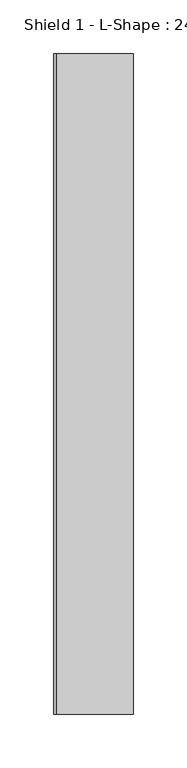
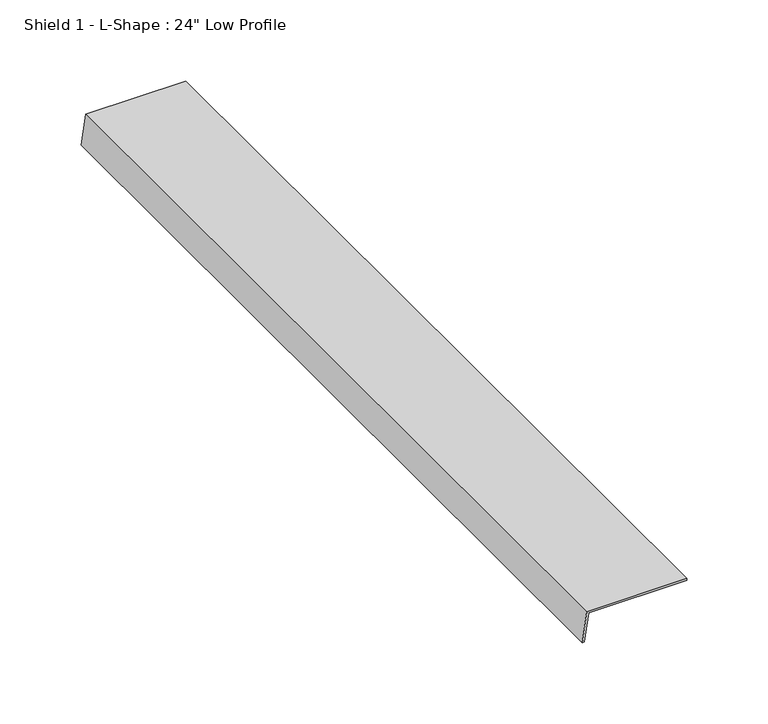
"""IFC4 building model written with IfcOpenShell, lengths in millimetres: proxy geometry."""

from ifc_helpers import new_model, si_unit, frame, origin, place, context, project, spatial, polyline, outline, extrude, source, transform, mapped, element, save


def proxy_87e85a14(model_context):
    return source(origin(), model_context, "Body", "SweptSolid", [
        extrude(outline(polyline([(22.225, -11.0820157), (0.0, -14.2570157), (0.0, -12.6695157), (20.6375, -9.4945157), (20.6375, 60.3554843), (22.225, 60.3554843), (22.225, -11.0820157)])), frame((0.0, -308.76875, 0.0), z_axis=(0.0, 1.0, 0.0), x_axis=(0.0, 0.0, 1.0)), (0.0, 0.0, 1.0), 617.5375),
    ])


if __name__ == "__main__":
    model = new_model("IFC4")
    model_context = context("Model", 3, world=origin())
    ifc_project = project(units=[si_unit("LENGTHUNIT", "METRE", prefix="MILLI")], contexts=[model_context])
    site = spatial("IfcSite", under=ifc_project)
    building = spatial("IfcBuilding", under=site)
    placement = place(None, origin())
    proxy_shape = proxy_87e85a14(model_context)
    element("IfcBuildingElementProxy", 1, Name="Shield 1 - L-Shape : 24\" Low Profile", ObjectType="Shield 1 - L-Shape : 24\" Low Profile", at=placement, inside=building, context=model_context, shape_type="MappedRepresentation", body=[
        mapped(proxy_shape, transform((0.0, 0.0, 0.0), x_axis=(1.0, 0.0, 0.0), y_axis=(0.0, 1.0, 0.0), z_axis=(0.0, 0.0, 1.0))),
    ])
    save(model, "model.ifc")

# Revit data of these elements
# Type "Shield 1 - L-Shape : 24\" Low Profile"
#   Type Comments = "⍁⍉⌁⌀⏭⎽⌇⍠⌜⍉⎖⌥⌦⌯⍭⏊⍻⍿⍊⏵⍊⏗⏠⍴⎡⌈⎀⍠⌓⌤⏘⎐⍀⌐⏬⏁⎈⏍⏦⎒⏬⌝⍩⍇⌣〈⎫〉⎁⏊⍥⍖⍥⍝⍦⌖⍀⏌⏭⎝⎼⏷⏞⍻⏯⎽⏷⏞⍻⏯⎽⏷⎺⌻⎝⍎⌧⏷⏟⏿⌿⍜⍦⍤⌁⍬⏶⏎⍊⏚⏉⎞⌡⎀⎪⏈⌟⌿⍾⍼⌟⌿⌢⍶⏯⏮⏭⏐⏿⍶⍷⏓⏻⎏⍶⌟⌼⏚⎹⎟⎾⏼⏢⏇⏎⎖⍭⍾⍑⍧⍭⌾⍋⍏〉⏺⍽⏙⎦⎯⎫⍲⏝⌖⏕⎲⏹⎱⎓⍪⍵⍝⌗⌗⏳⌶⎥⏗⍶⍆⏩⏙⏉⏫⌟⍻⍝⎝⎷⎳⏼⍷⍻⏻⏿"
#   URL = "http://www.metalux-lighting.com/"
#   Manufacturer = "Cooper Industries, Inc."
#   Width = 0' - 2 15/16"
#   Length = 2' - 0 7/16"
#   Height = 0' - 0 15/16"
#   CTRL Top Inset = 0' - 0 1/16"
#   CTRL Length = 2' - 0 5/16"
#   CTRL Housing Width = 0' - 5"
#   CTRL End Inset = 0' - 0 1/8"
#   Lens Material [instance default] = none
#   Assembly Code = ""
# Element 1 (IfcBuildingElementProxy, "Shield 1 - L-Shape : 24\" Low Profile")
#   Lens Material = Plastic - Cooper Industries - #12 Acrylic
#   Materials on its faces: "Plastic - Cooper Industries - #12 Acrylic"
# Materials
#   "Plastic - Cooper Industries - #12 Acrylic": class "Glass", colour RGB 249 250 249, transparency 0.8
